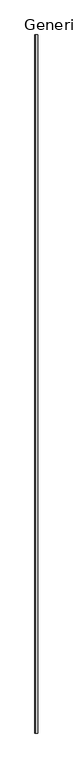
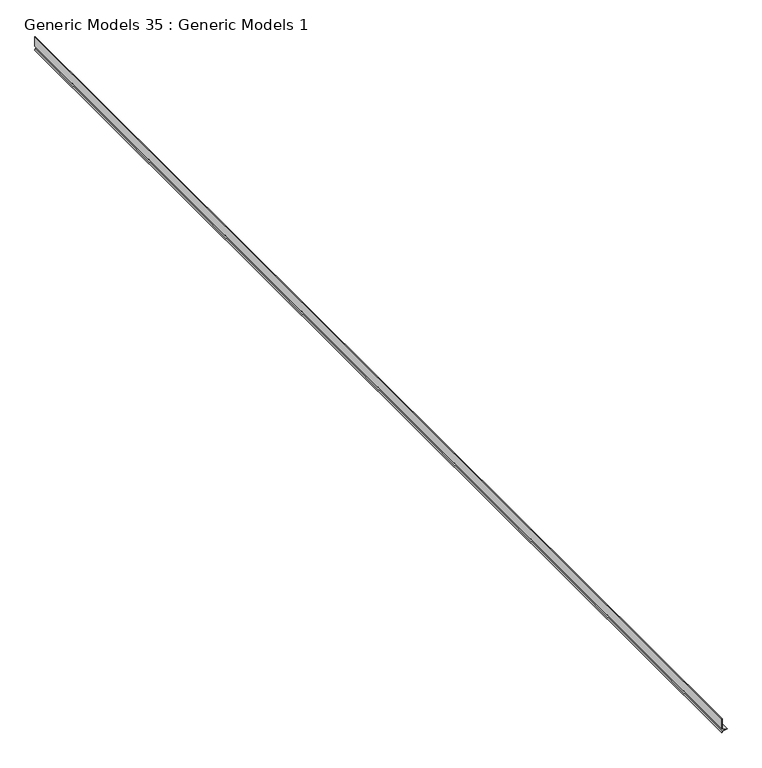
"""IFC4 building model written with IfcOpenShell, lengths in millimetres: proxy geometry, Generic Models 35 : Generic Models 1."""

from ifc_helpers import new_model, si_unit, origin, place, context, project, spatial, faceted_brep, source, transform, mapped, element, save


def generic_models_35_generic_models_1_29ce812b(model_context):
    return source(origin(), model_context, "Body", "Brep", [
        faceted_brep([(-9233.0736296, 11981.8769662, 126683.1304643), (-9253.2272461, 11981.8769662, 126676.6525161), (-9254.050567, 11981.8769662, 126672.2805244), (-9255.2986296, 11981.8769662, 126672.5155559), (-9254.3354345, 11981.8769662, 126677.6303063), (-9237.2238318, 11981.8769662, 126683.1304643), (-9255.2986296, 11981.8769662, 126688.9402207), (-9255.2986296, 11981.8769662, 126733.9304643), (-9254.0286296, 11981.8769662, 126733.9304643), (-9254.0286296, 11981.8769662, 126689.866), (-9248.4723795, 11981.8769662, 126688.0800625), (-9233.0736296, 6851.0769662, 126683.1304643), (-9254.0286296, 6851.0769662, 126689.866), (-9254.0286296, 6851.0769662, 126733.9304643), (-9255.2986296, 6851.0769662, 126733.9304643), (-9255.2986296, 6851.0769662, 126688.9402207), (-9237.2238318, 6851.0769662, 126683.1304643), (-9254.3354345, 6851.0769662, 126677.6303063), (-9255.2986296, 6851.0769662, 126672.5155559), (-9254.050567, 6851.0769662, 126672.2805244), (-9253.2272461, 6851.0769662, 126676.6525161)], [[[0, 1, 2, 3, 4, 5, 6, 7, 8, 9, 10]], [[11, 12, 13, 14, 15, 16, 17, 18, 19, 20]], [[0, 10, 9, 12, 11]], [[9, 8, 13, 12]], [[8, 7, 14, 13]], [[7, 6, 15, 14]], [[6, 5, 16, 15]], [[5, 4, 17, 16]], [[4, 3, 18, 17]], [[3, 2, 19, 18]], [[2, 1, 20, 19]], [[1, 0, 11, 20]]]),
    ])


if __name__ == "__main__":
    model = new_model("IFC4")
    model_context = context("Model", 3, world=origin())
    ifc_project = project(units=[si_unit("LENGTHUNIT", "METRE", prefix="MILLI")], contexts=[model_context])
    site = spatial("IfcSite", under=ifc_project)
    building = spatial("IfcBuilding", under=site)
    placement = place(None, origin())
    generic_models_35_generic_models_1_shape = generic_models_35_generic_models_1_29ce812b(model_context)
    element("IfcBuildingElementProxy", 1, Name="Generic Models 35 : Generic Models 1", ObjectType="Generic Models 35 : Generic Models 1", at=placement, inside=building, context=model_context, shape_type="MappedRepresentation", body=[
        mapped(generic_models_35_generic_models_1_shape, transform((0.0, 0.0, 0.0), x_axis=(1.0, 0.0, 0.0), y_axis=(0.0, 1.0, 0.0), z_axis=(0.0, 0.0, 1.0))),
    ])
    save(model, "model.ifc")

# Revit data of these elements
# Element 1 (IfcBuildingElementProxy, "Generic Models 35 : Generic Models 1")
#   Materials on its faces: "_16 GA. COPPER WEEP SCREED W/ MIN. 3 1/2\" ATTACHEMENT FLANGE - LAP UNDERLAYMENT OVER WEED SCREED"
# Materials
#   "_16 GA. COPPER WEEP SCREED W/ MIN. 3 1/2\" ATTACHEMENT FLANGE - LAP UNDERLAYMENT OVER WEED SCREED": class "Generic", colour RGB 253 192 103, transparency 0, Cost = 0
